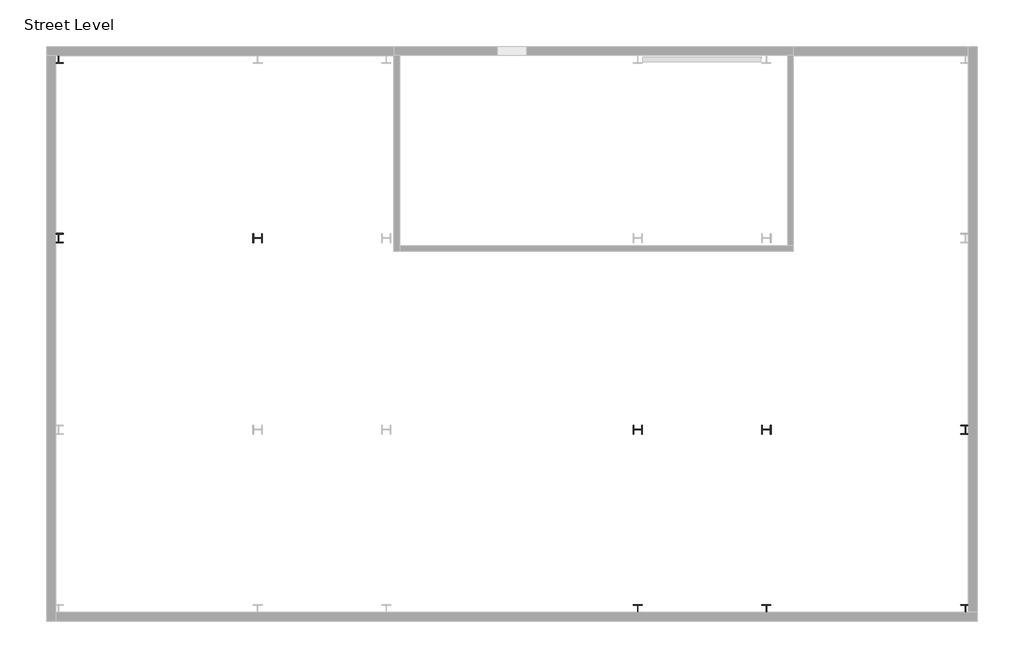
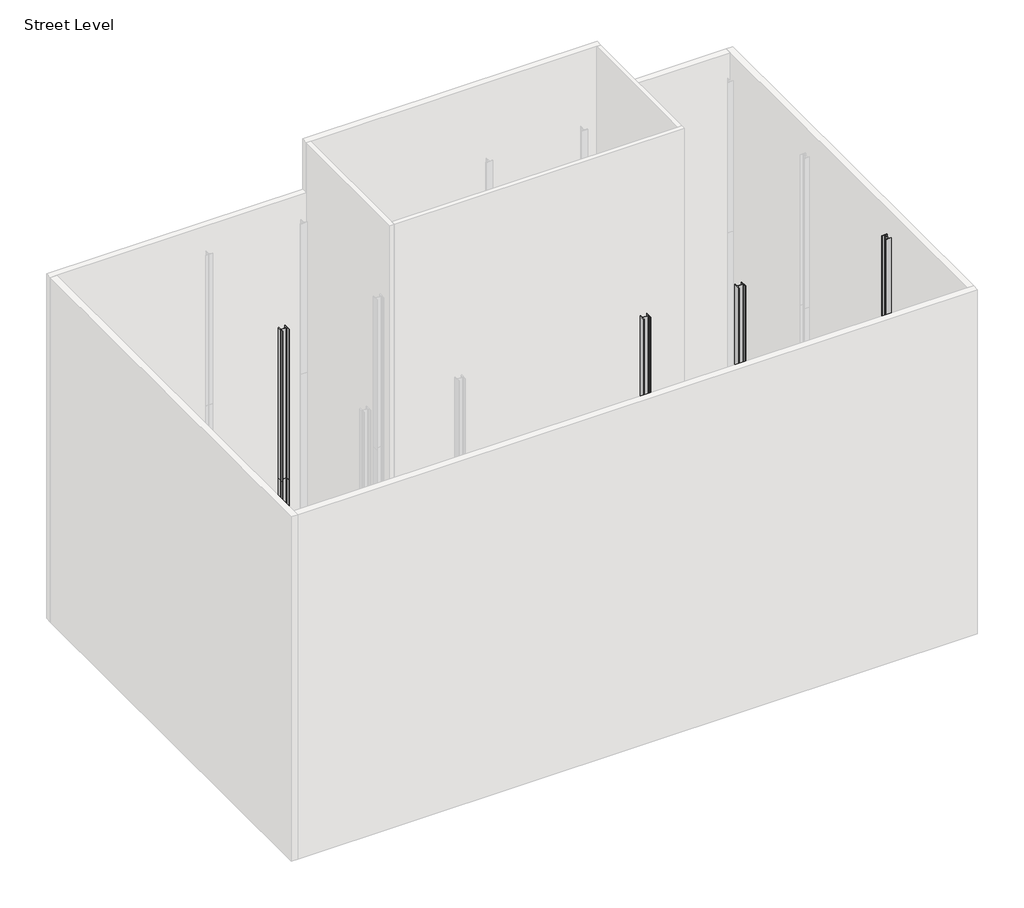
# One storey, part 2 of 3: 9 columns.
"""IFC4 building model written with IfcOpenShell, lengths in millimetres."""

from ifc_helpers import new_model, si_unit, point, frame, frame_2d, origin, place, context, project, spatial, polyline, circle_curve, trimmed, segment, composite_curve, outline, extrude, element, save

model = new_model("IFC4")

# Units and contexts
model_context = context("Model", 3, world=origin())
ifc_project = project(units=[si_unit("LENGTHUNIT", "METRE", prefix="MILLI")], contexts=[model_context])

# Site, building, storey
site = spatial("IfcSite", under=ifc_project)
building = spatial("IfcBuilding", under=site)
storey = spatial("IfcBuildingStorey", under=building, Name="Street Level", Elevation=-914.4)

# Columns
placement = place(None, origin())
element("IfcColumn", 1, ObjectType="W-Wide Flange-Column : W12X87", at=placement, inside=storey, context=model_context, shape_type="SweptSolid", body=[
    extrude(outline(composite_curve([segment(polyline([(3260.1377268, -3562.1684696), (3239.5637268, -3562.1684696), (3239.5637268, -3437.3274696)]), True, "CONTINUOUS"), segment(trimmed(circle_curve(frame_2d((3217.2752268, -3437.3274696)), 22.2885), [point((3239.5637268, -3437.3274696))], [point((3217.2752268, -3415.0389696))], True, "CARTESIAN"), True, "CONTINUOUS"), segment(polyline([(3217.2752268, -3415.0389696), (2985.5002268, -3415.0389696)]), True, "CONTINUOUS"), segment(trimmed(circle_curve(frame_2d((2985.5002268, -3437.3274696)), 22.2885), [point((2985.5002268, -3415.0389696))], [point((2963.2117268, -3437.3274696))], True, "CARTESIAN"), True, "CONTINUOUS"), segment(polyline([(2963.2117268, -3437.3274696), (2963.2117268, -3562.1684696), (2942.6377268, -3562.1684696), (2942.6377268, -3254.8284696), (2963.2117268, -3254.8284696), (2963.2117268, -3379.6694696)]), True, "CONTINUOUS"), segment(trimmed(circle_curve(frame_2d((2985.5002268, -3379.6694696)), 22.2885), [point((2963.2117268, -3379.6694696))], [point((2985.5002268, -3401.9579696))], True, "CARTESIAN"), True, "CONTINUOUS"), segment(polyline([(2985.5002268, -3401.9579696), (3217.2752268, -3401.9579696)]), True, "CONTINUOUS"), segment(trimmed(circle_curve(frame_2d((3217.2752268, -3379.6694696)), 22.2885), [point((3217.2752268, -3401.9579696))], [point((3239.5637268, -3379.6694696))], True, "CARTESIAN"), True, "CONTINUOUS"), segment(polyline([(3239.5637268, -3379.6694696), (3239.5637268, -3254.8284696), (3260.1377268, -3254.8284696), (3260.1377268, -3562.1684696)]), True, "CONTINUOUS")], self_intersect=False)), frame((0.0, 0.0, 7315.2), z_axis=(0.0, 0.0, 1.0), x_axis=(1.0, 0.0, 0.0)), (0.0, 0.0, 1.0), 7315.2),
    extrude(outline(composite_curve([segment(polyline([(3260.1377268, -3562.1684696), (3239.5637268, -3562.1684696), (3239.5637268, -3437.3274696)]), True, "CONTINUOUS"), segment(trimmed(circle_curve(frame_2d((3217.2752268, -3437.3274696)), 22.2885), [point((3239.5637268, -3437.3274696))], [point((3217.2752268, -3415.0389696))], True, "CARTESIAN"), True, "CONTINUOUS"), segment(polyline([(3217.2752268, -3415.0389696), (2985.5002268, -3415.0389696)]), True, "CONTINUOUS"), segment(trimmed(circle_curve(frame_2d((2985.5002268, -3437.3274696)), 22.2885), [point((2985.5002268, -3415.0389696))], [point((2963.2117268, -3437.3274696))], True, "CARTESIAN"), True, "CONTINUOUS"), segment(polyline([(2963.2117268, -3437.3274696), (2963.2117268, -3562.1684696), (2942.6377268, -3562.1684696), (2942.6377268, -3254.8284696), (2963.2117268, -3254.8284696), (2963.2117268, -3379.6694696)]), True, "CONTINUOUS"), segment(trimmed(circle_curve(frame_2d((2985.5002268, -3379.6694696)), 22.2885), [point((2963.2117268, -3379.6694696))], [point((2985.5002268, -3401.9579696))], True, "CARTESIAN"), True, "CONTINUOUS"), segment(polyline([(2985.5002268, -3401.9579696), (3217.2752268, -3401.9579696)]), True, "CONTINUOUS"), segment(trimmed(circle_curve(frame_2d((3217.2752268, -3379.6694696)), 22.2885), [point((3217.2752268, -3401.9579696))], [point((3239.5637268, -3379.6694696))], True, "CARTESIAN"), True, "CONTINUOUS"), segment(polyline([(3239.5637268, -3379.6694696), (3239.5637268, -3254.8284696), (3260.1377268, -3254.8284696), (3260.1377268, -3562.1684696)]), True, "CONTINUOUS")], self_intersect=False)), frame((0.0, 0.0, -914.4), z_axis=(0.0, 0.0, 1.0), x_axis=(1.0, 0.0, 0.0)), (0.0, 0.0, 1.0), 8229.6),
])
element("IfcColumn", 2, ObjectType="W-Wide Flange-Column : W12X87", at=placement, inside=storey, context=model_context, shape_type="SweptSolid", body=[
    extrude(outline(composite_curve([segment(polyline([(7628.9377268, -3562.1684696), (7608.3637268, -3562.1684696), (7608.3637268, -3437.3274696)]), True, "CONTINUOUS"), segment(trimmed(circle_curve(frame_2d((7586.0752268, -3437.3274696)), 22.2885), [point((7608.3637268, -3437.3274696))], [point((7586.0752268, -3415.0389696))], True, "CARTESIAN"), True, "CONTINUOUS"), segment(polyline([(7586.0752268, -3415.0389696), (7354.3002268, -3415.0389696)]), True, "CONTINUOUS"), segment(trimmed(circle_curve(frame_2d((7354.3002268, -3437.3274696)), 22.2885), [point((7354.3002268, -3415.0389696))], [point((7332.0117268, -3437.3274696))], True, "CARTESIAN"), True, "CONTINUOUS"), segment(polyline([(7332.0117268, -3437.3274696), (7332.0117268, -3562.1684696), (7311.4377268, -3562.1684696), (7311.4377268, -3254.8284696), (7332.0117268, -3254.8284696), (7332.0117268, -3379.6694696)]), True, "CONTINUOUS"), segment(trimmed(circle_curve(frame_2d((7354.3002268, -3379.6694696)), 22.2885), [point((7332.0117268, -3379.6694696))], [point((7354.3002268, -3401.9579696))], True, "CARTESIAN"), True, "CONTINUOUS"), segment(polyline([(7354.3002268, -3401.9579696), (7586.0752268, -3401.9579696)]), True, "CONTINUOUS"), segment(trimmed(circle_curve(frame_2d((7586.0752268, -3379.6694696)), 22.2885), [point((7586.0752268, -3401.9579696))], [point((7608.3637268, -3379.6694696))], True, "CARTESIAN"), True, "CONTINUOUS"), segment(polyline([(7608.3637268, -3379.6694696), (7608.3637268, -3254.8284696), (7628.9377268, -3254.8284696), (7628.9377268, -3562.1684696)]), True, "CONTINUOUS")], self_intersect=False)), frame((0.0, 0.0, 7315.2), z_axis=(0.0, 0.0, 1.0), x_axis=(1.0, 0.0, 0.0)), (0.0, 0.0, 1.0), 7315.2),
    extrude(outline(composite_curve([segment(polyline([(7628.9377268, -3562.1684696), (7608.3637268, -3562.1684696), (7608.3637268, -3437.3274696)]), True, "CONTINUOUS"), segment(trimmed(circle_curve(frame_2d((7586.0752268, -3437.3274696)), 22.2885), [point((7608.3637268, -3437.3274696))], [point((7586.0752268, -3415.0389696))], True, "CARTESIAN"), True, "CONTINUOUS"), segment(polyline([(7586.0752268, -3415.0389696), (7354.3002268, -3415.0389696)]), True, "CONTINUOUS"), segment(trimmed(circle_curve(frame_2d((7354.3002268, -3437.3274696)), 22.2885), [point((7354.3002268, -3415.0389696))], [point((7332.0117268, -3437.3274696))], True, "CARTESIAN"), True, "CONTINUOUS"), segment(polyline([(7332.0117268, -3437.3274696), (7332.0117268, -3562.1684696), (7311.4377268, -3562.1684696), (7311.4377268, -3254.8284696), (7332.0117268, -3254.8284696), (7332.0117268, -3379.6694696)]), True, "CONTINUOUS"), segment(trimmed(circle_curve(frame_2d((7354.3002268, -3379.6694696)), 22.2885), [point((7332.0117268, -3379.6694696))], [point((7354.3002268, -3401.9579696))], True, "CARTESIAN"), True, "CONTINUOUS"), segment(polyline([(7354.3002268, -3401.9579696), (7586.0752268, -3401.9579696)]), True, "CONTINUOUS"), segment(trimmed(circle_curve(frame_2d((7586.0752268, -3379.6694696)), 22.2885), [point((7586.0752268, -3401.9579696))], [point((7608.3637268, -3379.6694696))], True, "CARTESIAN"), True, "CONTINUOUS"), segment(polyline([(7608.3637268, -3379.6694696), (7608.3637268, -3254.8284696), (7628.9377268, -3254.8284696), (7628.9377268, -3562.1684696)]), True, "CONTINUOUS")], self_intersect=False)), frame((0.0, 0.0, -914.4), z_axis=(0.0, 0.0, 1.0), x_axis=(1.0, 0.0, 0.0)), (0.0, 0.0, 1.0), 8229.6),
])
element("IfcColumn", 3, ObjectType="W-Wide Flange-Column : W12X87", at=placement, inside=storey, context=model_context, shape_type="SweptSolid", body=[
    extrude(outline(composite_curve([segment(polyline([(-9643.0622732, 2940.2315304), (-9663.6362732, 2940.2315304), (-9663.6362732, 3065.0725304)]), True, "CONTINUOUS"), segment(trimmed(circle_curve(frame_2d((-9685.9247732, 3065.0725304)), 22.2885), [point((-9663.6362732, 3065.0725304))], [point((-9685.9247732, 3087.3610304))], True, "CARTESIAN"), True, "CONTINUOUS"), segment(polyline([(-9685.9247732, 3087.3610304), (-9917.6997732, 3087.3610304)]), True, "CONTINUOUS"), segment(trimmed(circle_curve(frame_2d((-9917.6997732, 3065.0725304)), 22.2885), [point((-9917.6997732, 3087.3610304))], [point((-9939.9882732, 3065.0725304))], True, "CARTESIAN"), True, "CONTINUOUS"), segment(polyline([(-9939.9882732, 3065.0725304), (-9939.9882732, 2940.2315304), (-9960.5622732, 2940.2315304), (-9960.5622732, 3247.5715304), (-9939.9882732, 3247.5715304), (-9939.9882732, 3122.7305304)]), True, "CONTINUOUS"), segment(trimmed(circle_curve(frame_2d((-9917.6997732, 3122.7305304)), 22.2885), [point((-9939.9882732, 3122.7305304))], [point((-9917.6997732, 3100.4420304))], True, "CARTESIAN"), True, "CONTINUOUS"), segment(polyline([(-9917.6997732, 3100.4420304), (-9685.9247732, 3100.4420304)]), True, "CONTINUOUS"), segment(trimmed(circle_curve(frame_2d((-9685.9247732, 3122.7305304)), 22.2885), [point((-9685.9247732, 3100.4420304))], [point((-9663.6362732, 3122.7305304))], True, "CARTESIAN"), True, "CONTINUOUS"), segment(polyline([(-9663.6362732, 3122.7305304), (-9663.6362732, 3247.5715304), (-9643.0622732, 3247.5715304), (-9643.0622732, 2940.2315304)]), True, "CONTINUOUS")], self_intersect=False)), frame((0.0, 0.0, 7315.2), z_axis=(0.0, 0.0, 1.0), x_axis=(1.0, 0.0, 0.0)), (0.0, 0.0, 1.0), 7315.2),
    extrude(outline(composite_curve([segment(polyline([(-9643.0622732, 2940.2315304), (-9663.6362732, 2940.2315304), (-9663.6362732, 3065.0725304)]), True, "CONTINUOUS"), segment(trimmed(circle_curve(frame_2d((-9685.9247732, 3065.0725304)), 22.2885), [point((-9663.6362732, 3065.0725304))], [point((-9685.9247732, 3087.3610304))], True, "CARTESIAN"), True, "CONTINUOUS"), segment(polyline([(-9685.9247732, 3087.3610304), (-9917.6997732, 3087.3610304)]), True, "CONTINUOUS"), segment(trimmed(circle_curve(frame_2d((-9917.6997732, 3065.0725304)), 22.2885), [point((-9917.6997732, 3087.3610304))], [point((-9939.9882732, 3065.0725304))], True, "CARTESIAN"), True, "CONTINUOUS"), segment(polyline([(-9939.9882732, 3065.0725304), (-9939.9882732, 2940.2315304), (-9960.5622732, 2940.2315304), (-9960.5622732, 3247.5715304), (-9939.9882732, 3247.5715304), (-9939.9882732, 3122.7305304)]), True, "CONTINUOUS"), segment(trimmed(circle_curve(frame_2d((-9917.6997732, 3122.7305304)), 22.2885), [point((-9939.9882732, 3122.7305304))], [point((-9917.6997732, 3100.4420304))], True, "CARTESIAN"), True, "CONTINUOUS"), segment(polyline([(-9917.6997732, 3100.4420304), (-9685.9247732, 3100.4420304)]), True, "CONTINUOUS"), segment(trimmed(circle_curve(frame_2d((-9685.9247732, 3122.7305304)), 22.2885), [point((-9685.9247732, 3100.4420304))], [point((-9663.6362732, 3122.7305304))], True, "CARTESIAN"), True, "CONTINUOUS"), segment(polyline([(-9663.6362732, 3122.7305304), (-9663.6362732, 3247.5715304), (-9643.0622732, 3247.5715304), (-9643.0622732, 2940.2315304)]), True, "CONTINUOUS")], self_intersect=False)), frame((0.0, 0.0, -914.4), z_axis=(0.0, 0.0, 1.0), x_axis=(1.0, 0.0, 0.0)), (0.0, 0.0, 1.0), 8229.6),
])
element("IfcColumn", 4, ObjectType="W-Wide Flange-Column : W12X87", at=placement, inside=storey, context=model_context, shape_type="SweptSolid", body=[
    extrude(outline(composite_curve([segment(polyline([(-16404.5422732, 9348.6515304), (-16404.5422732, 9328.0775304), (-16529.3832732, 9328.0775304)]), True, "CONTINUOUS"), segment(trimmed(circle_curve(frame_2d((-16529.3832732, 9305.7890304)), 22.2885), [point((-16529.3832732, 9328.0775304))], [point((-16551.6717732, 9305.7890304))], True, "CARTESIAN"), True, "CONTINUOUS"), segment(polyline([(-16551.6717732, 9305.7890304), (-16551.6717732, 9074.0140304)]), True, "CONTINUOUS"), segment(trimmed(circle_curve(frame_2d((-16529.3832732, 9074.0140304)), 22.2885), [point((-16551.6717732, 9074.0140304))], [point((-16529.3832732, 9051.7255304))], True, "CARTESIAN"), True, "CONTINUOUS"), segment(polyline([(-16529.3832732, 9051.7255304), (-16404.5422732, 9051.7255304), (-16404.5422732, 9031.1515304), (-16711.8822732, 9031.1515304), (-16711.8822732, 9051.7255304), (-16587.0412732, 9051.7255304)]), True, "CONTINUOUS"), segment(trimmed(circle_curve(frame_2d((-16587.0412732, 9074.0140304)), 22.2885), [point((-16587.0412732, 9051.7255304))], [point((-16564.7527732, 9074.0140304))], True, "CARTESIAN"), True, "CONTINUOUS"), segment(polyline([(-16564.7527732, 9074.0140304), (-16564.7527732, 9305.7890304)]), True, "CONTINUOUS"), segment(trimmed(circle_curve(frame_2d((-16587.0412732, 9305.7890304)), 22.2885), [point((-16564.7527732, 9305.7890304))], [point((-16587.0412732, 9328.0775304))], True, "CARTESIAN"), True, "CONTINUOUS"), segment(polyline([(-16587.0412732, 9328.0775304), (-16711.8822732, 9328.0775304), (-16711.8822732, 9348.6515304), (-16404.5422732, 9348.6515304)]), True, "CONTINUOUS")], self_intersect=False)), frame((0.0, 0.0, 7315.2), z_axis=(0.0, 0.0, 1.0), x_axis=(1.0, 0.0, 0.0)), (0.0, 0.0, 1.0), 7315.2),
    extrude(outline(composite_curve([segment(polyline([(-16404.5422732, 9348.6515304), (-16404.5422732, 9328.0775304), (-16529.3832732, 9328.0775304)]), True, "CONTINUOUS"), segment(trimmed(circle_curve(frame_2d((-16529.3832732, 9305.7890304)), 22.2885), [point((-16529.3832732, 9328.0775304))], [point((-16551.6717732, 9305.7890304))], True, "CARTESIAN"), True, "CONTINUOUS"), segment(polyline([(-16551.6717732, 9305.7890304), (-16551.6717732, 9074.0140304)]), True, "CONTINUOUS"), segment(trimmed(circle_curve(frame_2d((-16529.3832732, 9074.0140304)), 22.2885), [point((-16551.6717732, 9074.0140304))], [point((-16529.3832732, 9051.7255304))], True, "CARTESIAN"), True, "CONTINUOUS"), segment(polyline([(-16529.3832732, 9051.7255304), (-16404.5422732, 9051.7255304), (-16404.5422732, 9031.1515304), (-16711.8822732, 9031.1515304), (-16711.8822732, 9051.7255304), (-16587.0412732, 9051.7255304)]), True, "CONTINUOUS"), segment(trimmed(circle_curve(frame_2d((-16587.0412732, 9074.0140304)), 22.2885), [point((-16587.0412732, 9051.7255304))], [point((-16564.7527732, 9074.0140304))], True, "CARTESIAN"), True, "CONTINUOUS"), segment(polyline([(-16564.7527732, 9074.0140304), (-16564.7527732, 9305.7890304)]), True, "CONTINUOUS"), segment(trimmed(circle_curve(frame_2d((-16587.0412732, 9305.7890304)), 22.2885), [point((-16564.7527732, 9305.7890304))], [point((-16587.0412732, 9328.0775304))], True, "CARTESIAN"), True, "CONTINUOUS"), segment(polyline([(-16587.0412732, 9328.0775304), (-16711.8822732, 9328.0775304), (-16711.8822732, 9348.6515304), (-16404.5422732, 9348.6515304)]), True, "CONTINUOUS")], self_intersect=False)), frame((0.0, 0.0, -914.4), z_axis=(0.0, 0.0, 1.0), x_axis=(1.0, 0.0, 0.0)), (0.0, 0.0, 1.0), 8229.6),
])
element("IfcColumn", 5, ObjectType="W-Wide Flange-Column : W12X87", at=placement, inside=storey, context=model_context, shape_type="SweptSolid", body=[
    extrude(outline(composite_curve([segment(polyline([(-16404.5422732, 3252.6515304), (-16404.5422732, 3232.0775304), (-16529.3832732, 3232.0775304)]), True, "CONTINUOUS"), segment(trimmed(circle_curve(frame_2d((-16529.3832732, 3209.7890304)), 22.2885), [point((-16529.3832732, 3232.0775304))], [point((-16551.6717732, 3209.7890304))], True, "CARTESIAN"), True, "CONTINUOUS"), segment(polyline([(-16551.6717732, 3209.7890304), (-16551.6717732, 2978.0140304)]), True, "CONTINUOUS"), segment(trimmed(circle_curve(frame_2d((-16529.3832732, 2978.0140304)), 22.2885), [point((-16551.6717732, 2978.0140304))], [point((-16529.3832732, 2955.7255304))], True, "CARTESIAN"), True, "CONTINUOUS"), segment(polyline([(-16529.3832732, 2955.7255304), (-16404.5422732, 2955.7255304), (-16404.5422732, 2935.1515304), (-16711.8822732, 2935.1515304), (-16711.8822732, 2955.7255304), (-16587.0412732, 2955.7255304)]), True, "CONTINUOUS"), segment(trimmed(circle_curve(frame_2d((-16587.0412732, 2978.0140304)), 22.2885), [point((-16587.0412732, 2955.7255304))], [point((-16564.7527732, 2978.0140304))], True, "CARTESIAN"), True, "CONTINUOUS"), segment(polyline([(-16564.7527732, 2978.0140304), (-16564.7527732, 3209.7890304)]), True, "CONTINUOUS"), segment(trimmed(circle_curve(frame_2d((-16587.0412732, 3209.7890304)), 22.2885), [point((-16564.7527732, 3209.7890304))], [point((-16587.0412732, 3232.0775304))], True, "CARTESIAN"), True, "CONTINUOUS"), segment(polyline([(-16587.0412732, 3232.0775304), (-16711.8822732, 3232.0775304), (-16711.8822732, 3252.6515304), (-16404.5422732, 3252.6515304)]), True, "CONTINUOUS")], self_intersect=False)), frame((0.0, 0.0, 7315.2), z_axis=(0.0, 0.0, 1.0), x_axis=(1.0, 0.0, 0.0)), (0.0, 0.0, 1.0), 7315.2),
    extrude(outline(composite_curve([segment(polyline([(-16404.5422732, 3252.6515304), (-16404.5422732, 3232.0775304), (-16529.3832732, 3232.0775304)]), True, "CONTINUOUS"), segment(trimmed(circle_curve(frame_2d((-16529.3832732, 3209.7890304)), 22.2885), [point((-16529.3832732, 3232.0775304))], [point((-16551.6717732, 3209.7890304))], True, "CARTESIAN"), True, "CONTINUOUS"), segment(polyline([(-16551.6717732, 3209.7890304), (-16551.6717732, 2978.0140304)]), True, "CONTINUOUS"), segment(trimmed(circle_curve(frame_2d((-16529.3832732, 2978.0140304)), 22.2885), [point((-16551.6717732, 2978.0140304))], [point((-16529.3832732, 2955.7255304))], True, "CARTESIAN"), True, "CONTINUOUS"), segment(polyline([(-16529.3832732, 2955.7255304), (-16404.5422732, 2955.7255304), (-16404.5422732, 2935.1515304), (-16711.8822732, 2935.1515304), (-16711.8822732, 2955.7255304), (-16587.0412732, 2955.7255304)]), True, "CONTINUOUS"), segment(trimmed(circle_curve(frame_2d((-16587.0412732, 2978.0140304)), 22.2885), [point((-16587.0412732, 2955.7255304))], [point((-16564.7527732, 2978.0140304))], True, "CARTESIAN"), True, "CONTINUOUS"), segment(polyline([(-16564.7527732, 2978.0140304), (-16564.7527732, 3209.7890304)]), True, "CONTINUOUS"), segment(trimmed(circle_curve(frame_2d((-16587.0412732, 3209.7890304)), 22.2885), [point((-16564.7527732, 3209.7890304))], [point((-16587.0412732, 3232.0775304))], True, "CARTESIAN"), True, "CONTINUOUS"), segment(polyline([(-16587.0412732, 3232.0775304), (-16711.8822732, 3232.0775304), (-16711.8822732, 3252.6515304), (-16404.5422732, 3252.6515304)]), True, "CONTINUOUS")], self_intersect=False)), frame((0.0, 0.0, -914.4), z_axis=(0.0, 0.0, 1.0), x_axis=(1.0, 0.0, 0.0)), (0.0, 0.0, 1.0), 8229.6),
])
element("IfcColumn", 6, ObjectType="W-Wide Flange-Column : W12X87", at=placement, inside=storey, context=model_context, shape_type="SweptSolid", body=[
    extrude(outline(composite_curve([segment(polyline([(14380.2577268, -3249.7484696), (14380.2577268, -3270.3224696), (14255.4167268, -3270.3224696)]), True, "CONTINUOUS"), segment(trimmed(circle_curve(frame_2d((14255.4167268, -3292.6109696)), 22.2885), [point((14255.4167268, -3270.3224696))], [point((14233.1282268, -3292.6109696))], True, "CARTESIAN"), True, "CONTINUOUS"), segment(polyline([(14233.1282268, -3292.6109696), (14233.1282268, -3524.3859696)]), True, "CONTINUOUS"), segment(trimmed(circle_curve(frame_2d((14255.4167268, -3524.3859696)), 22.2885), [point((14233.1282268, -3524.3859696))], [point((14255.4167268, -3546.6744696))], True, "CARTESIAN"), True, "CONTINUOUS"), segment(polyline([(14255.4167268, -3546.6744696), (14380.2577268, -3546.6744696), (14380.2577268, -3567.2484696), (14072.9177268, -3567.2484696), (14072.9177268, -3546.6744696), (14197.7587268, -3546.6744696)]), True, "CONTINUOUS"), segment(trimmed(circle_curve(frame_2d((14197.7587268, -3524.3859696)), 22.2885), [point((14197.7587268, -3546.6744696))], [point((14220.0472268, -3524.3859696))], True, "CARTESIAN"), True, "CONTINUOUS"), segment(polyline([(14220.0472268, -3524.3859696), (14220.0472268, -3292.6109696)]), True, "CONTINUOUS"), segment(trimmed(circle_curve(frame_2d((14197.7587268, -3292.6109696)), 22.2885), [point((14220.0472268, -3292.6109696))], [point((14197.7587268, -3270.3224696))], True, "CARTESIAN"), True, "CONTINUOUS"), segment(polyline([(14197.7587268, -3270.3224696), (14072.9177268, -3270.3224696), (14072.9177268, -3249.7484696), (14380.2577268, -3249.7484696)]), True, "CONTINUOUS")], self_intersect=False)), frame((0.0, 0.0, 7315.2), z_axis=(0.0, 0.0, 1.0), x_axis=(1.0, 0.0, 0.0)), (0.0, 0.0, 1.0), 7315.2),
    extrude(outline(composite_curve([segment(polyline([(14380.2577268, -3249.7484696), (14380.2577268, -3270.3224696), (14255.4167268, -3270.3224696)]), True, "CONTINUOUS"), segment(trimmed(circle_curve(frame_2d((14255.4167268, -3292.6109696)), 22.2885), [point((14255.4167268, -3270.3224696))], [point((14233.1282268, -3292.6109696))], True, "CARTESIAN"), True, "CONTINUOUS"), segment(polyline([(14233.1282268, -3292.6109696), (14233.1282268, -3524.3859696)]), True, "CONTINUOUS"), segment(trimmed(circle_curve(frame_2d((14255.4167268, -3524.3859696)), 22.2885), [point((14233.1282268, -3524.3859696))], [point((14255.4167268, -3546.6744696))], True, "CARTESIAN"), True, "CONTINUOUS"), segment(polyline([(14255.4167268, -3546.6744696), (14380.2577268, -3546.6744696), (14380.2577268, -3567.2484696), (14072.9177268, -3567.2484696), (14072.9177268, -3546.6744696), (14197.7587268, -3546.6744696)]), True, "CONTINUOUS"), segment(trimmed(circle_curve(frame_2d((14197.7587268, -3524.3859696)), 22.2885), [point((14197.7587268, -3546.6744696))], [point((14220.0472268, -3524.3859696))], True, "CARTESIAN"), True, "CONTINUOUS"), segment(polyline([(14220.0472268, -3524.3859696), (14220.0472268, -3292.6109696)]), True, "CONTINUOUS"), segment(trimmed(circle_curve(frame_2d((14197.7587268, -3292.6109696)), 22.2885), [point((14220.0472268, -3292.6109696))], [point((14197.7587268, -3270.3224696))], True, "CARTESIAN"), True, "CONTINUOUS"), segment(polyline([(14197.7587268, -3270.3224696), (14072.9177268, -3270.3224696), (14072.9177268, -3249.7484696), (14380.2577268, -3249.7484696)]), True, "CONTINUOUS")], self_intersect=False)), frame((0.0, 0.0, -914.4), z_axis=(0.0, 0.0, 1.0), x_axis=(1.0, 0.0, 0.0)), (0.0, 0.0, 1.0), 8229.6),
])
element("IfcColumn", 7, ObjectType="W-Wide Flange-Column : W12X87", at=placement, inside=storey, context=model_context, shape_type="SweptSolid", body=[
    extrude(outline(composite_curve([segment(polyline([(14380.2577268, -9345.7484696), (14380.2577268, -9366.3224696), (14255.4167268, -9366.3224696)]), True, "CONTINUOUS"), segment(trimmed(circle_curve(frame_2d((14255.4167268, -9388.6109696)), 22.2885), [point((14255.4167268, -9366.3224696))], [point((14233.1282268, -9388.6109696))], True, "CARTESIAN"), True, "CONTINUOUS"), segment(polyline([(14233.1282268, -9388.6109696), (14233.1282268, -9620.3859696)]), True, "CONTINUOUS"), segment(trimmed(circle_curve(frame_2d((14255.4167268, -9620.3859696)), 22.2885), [point((14233.1282268, -9620.3859696))], [point((14255.4167268, -9642.6744696))], True, "CARTESIAN"), True, "CONTINUOUS"), segment(polyline([(14255.4167268, -9642.6744696), (14380.2577268, -9642.6744696), (14380.2577268, -9663.2484696), (14072.9177268, -9663.2484696), (14072.9177268, -9642.6744696), (14197.7587268, -9642.6744696)]), True, "CONTINUOUS"), segment(trimmed(circle_curve(frame_2d((14197.7587268, -9620.3859696)), 22.2885), [point((14197.7587268, -9642.6744696))], [point((14220.0472268, -9620.3859696))], True, "CARTESIAN"), True, "CONTINUOUS"), segment(polyline([(14220.0472268, -9620.3859696), (14220.0472268, -9388.6109696)]), True, "CONTINUOUS"), segment(trimmed(circle_curve(frame_2d((14197.7587268, -9388.6109696)), 22.2885), [point((14220.0472268, -9388.6109696))], [point((14197.7587268, -9366.3224696))], True, "CARTESIAN"), True, "CONTINUOUS"), segment(polyline([(14197.7587268, -9366.3224696), (14072.9177268, -9366.3224696), (14072.9177268, -9345.7484696), (14380.2577268, -9345.7484696)]), True, "CONTINUOUS")], self_intersect=False)), frame((0.0, 0.0, 7315.2), z_axis=(0.0, 0.0, 1.0), x_axis=(1.0, 0.0, 0.0)), (0.0, 0.0, 1.0), 7315.2),
    extrude(outline(composite_curve([segment(polyline([(14380.2577268, -9345.7484696), (14380.2577268, -9366.3224696), (14255.4167268, -9366.3224696)]), True, "CONTINUOUS"), segment(trimmed(circle_curve(frame_2d((14255.4167268, -9388.6109696)), 22.2885), [point((14255.4167268, -9366.3224696))], [point((14233.1282268, -9388.6109696))], True, "CARTESIAN"), True, "CONTINUOUS"), segment(polyline([(14233.1282268, -9388.6109696), (14233.1282268, -9620.3859696)]), True, "CONTINUOUS"), segment(trimmed(circle_curve(frame_2d((14255.4167268, -9620.3859696)), 22.2885), [point((14233.1282268, -9620.3859696))], [point((14255.4167268, -9642.6744696))], True, "CARTESIAN"), True, "CONTINUOUS"), segment(polyline([(14255.4167268, -9642.6744696), (14380.2577268, -9642.6744696), (14380.2577268, -9663.2484696), (14072.9177268, -9663.2484696), (14072.9177268, -9642.6744696), (14197.7587268, -9642.6744696)]), True, "CONTINUOUS"), segment(trimmed(circle_curve(frame_2d((14197.7587268, -9620.3859696)), 22.2885), [point((14197.7587268, -9642.6744696))], [point((14220.0472268, -9620.3859696))], True, "CARTESIAN"), True, "CONTINUOUS"), segment(polyline([(14220.0472268, -9620.3859696), (14220.0472268, -9388.6109696)]), True, "CONTINUOUS"), segment(trimmed(circle_curve(frame_2d((14197.7587268, -9388.6109696)), 22.2885), [point((14220.0472268, -9388.6109696))], [point((14197.7587268, -9366.3224696))], True, "CARTESIAN"), True, "CONTINUOUS"), segment(polyline([(14197.7587268, -9366.3224696), (14072.9177268, -9366.3224696), (14072.9177268, -9345.7484696), (14380.2577268, -9345.7484696)]), True, "CONTINUOUS")], self_intersect=False)), frame((0.0, 0.0, -914.4), z_axis=(0.0, 0.0, 1.0), x_axis=(1.0, 0.0, 0.0)), (0.0, 0.0, 1.0), 8229.6),
])
element("IfcColumn", 8, ObjectType="W-Wide Flange-Column : W12X87", at=placement, inside=storey, context=model_context, shape_type="SweptSolid", body=[
    extrude(outline(composite_curve([segment(polyline([(7623.8577268, -9345.7484696), (7623.8577268, -9366.3224696), (7499.0167268, -9366.3224696)]), True, "CONTINUOUS"), segment(trimmed(circle_curve(frame_2d((7499.0167268, -9388.6109696)), 22.2885), [point((7499.0167268, -9366.3224696))], [point((7476.7282268, -9388.6109696))], True, "CARTESIAN"), True, "CONTINUOUS"), segment(polyline([(7476.7282268, -9388.6109696), (7476.7282268, -9620.3859696)]), True, "CONTINUOUS"), segment(trimmed(circle_curve(frame_2d((7499.0167268, -9620.3859696)), 22.2885), [point((7476.7282268, -9620.3859696))], [point((7499.0167268, -9642.6744696))], True, "CARTESIAN"), True, "CONTINUOUS"), segment(polyline([(7499.0167268, -9642.6744696), (7623.8577268, -9642.6744696), (7623.8577268, -9663.2484696), (7316.5177268, -9663.2484696), (7316.5177268, -9642.6744696), (7441.3587268, -9642.6744696)]), True, "CONTINUOUS"), segment(trimmed(circle_curve(frame_2d((7441.3587268, -9620.3859696)), 22.2885), [point((7441.3587268, -9642.6744696))], [point((7463.6472268, -9620.3859696))], True, "CARTESIAN"), True, "CONTINUOUS"), segment(polyline([(7463.6472268, -9620.3859696), (7463.6472268, -9388.6109696)]), True, "CONTINUOUS"), segment(trimmed(circle_curve(frame_2d((7441.3587268, -9388.6109696)), 22.2885), [point((7463.6472268, -9388.6109696))], [point((7441.3587268, -9366.3224696))], True, "CARTESIAN"), True, "CONTINUOUS"), segment(polyline([(7441.3587268, -9366.3224696), (7316.5177268, -9366.3224696), (7316.5177268, -9345.7484696), (7623.8577268, -9345.7484696)]), True, "CONTINUOUS")], self_intersect=False)), frame((0.0, 0.0, 7315.2), z_axis=(0.0, 0.0, 1.0), x_axis=(1.0, 0.0, 0.0)), (0.0, 0.0, 1.0), 7315.2),
    extrude(outline(composite_curve([segment(polyline([(7623.8577268, -9345.7484696), (7623.8577268, -9366.3224696), (7499.0167268, -9366.3224696)]), True, "CONTINUOUS"), segment(trimmed(circle_curve(frame_2d((7499.0167268, -9388.6109696)), 22.2885), [point((7499.0167268, -9366.3224696))], [point((7476.7282268, -9388.6109696))], True, "CARTESIAN"), True, "CONTINUOUS"), segment(polyline([(7476.7282268, -9388.6109696), (7476.7282268, -9620.3859696)]), True, "CONTINUOUS"), segment(trimmed(circle_curve(frame_2d((7499.0167268, -9620.3859696)), 22.2885), [point((7476.7282268, -9620.3859696))], [point((7499.0167268, -9642.6744696))], True, "CARTESIAN"), True, "CONTINUOUS"), segment(polyline([(7499.0167268, -9642.6744696), (7623.8577268, -9642.6744696), (7623.8577268, -9663.2484696), (7316.5177268, -9663.2484696), (7316.5177268, -9642.6744696), (7441.3587268, -9642.6744696)]), True, "CONTINUOUS"), segment(trimmed(circle_curve(frame_2d((7441.3587268, -9620.3859696)), 22.2885), [point((7441.3587268, -9642.6744696))], [point((7463.6472268, -9620.3859696))], True, "CARTESIAN"), True, "CONTINUOUS"), segment(polyline([(7463.6472268, -9620.3859696), (7463.6472268, -9388.6109696)]), True, "CONTINUOUS"), segment(trimmed(circle_curve(frame_2d((7441.3587268, -9388.6109696)), 22.2885), [point((7463.6472268, -9388.6109696))], [point((7441.3587268, -9366.3224696))], True, "CARTESIAN"), True, "CONTINUOUS"), segment(polyline([(7441.3587268, -9366.3224696), (7316.5177268, -9366.3224696), (7316.5177268, -9345.7484696), (7623.8577268, -9345.7484696)]), True, "CONTINUOUS")], self_intersect=False)), frame((0.0, 0.0, -914.4), z_axis=(0.0, 0.0, 1.0), x_axis=(1.0, 0.0, 0.0)), (0.0, 0.0, 1.0), 8229.6),
])
element("IfcColumn", 9, ObjectType="W-Wide Flange-Column : W12X87", at=placement, inside=storey, context=model_context, shape_type="SweptSolid", body=[
    extrude(outline(composite_curve([segment(polyline([(3255.0577268, -9345.7484696), (3255.0577268, -9366.3224696), (3130.2167268, -9366.3224696)]), True, "CONTINUOUS"), segment(trimmed(circle_curve(frame_2d((3130.2167268, -9388.6109696)), 22.2885), [point((3130.2167268, -9366.3224696))], [point((3107.9282268, -9388.6109696))], True, "CARTESIAN"), True, "CONTINUOUS"), segment(polyline([(3107.9282268, -9388.6109696), (3107.9282268, -9620.3859696)]), True, "CONTINUOUS"), segment(trimmed(circle_curve(frame_2d((3130.2167268, -9620.3859696)), 22.2885), [point((3107.9282268, -9620.3859696))], [point((3130.2167268, -9642.6744696))], True, "CARTESIAN"), True, "CONTINUOUS"), segment(polyline([(3130.2167268, -9642.6744696), (3255.0577268, -9642.6744696), (3255.0577268, -9663.2484696), (2947.7177268, -9663.2484696), (2947.7177268, -9642.6744696), (3072.5587268, -9642.6744696)]), True, "CONTINUOUS"), segment(trimmed(circle_curve(frame_2d((3072.5587268, -9620.3859696)), 22.2885), [point((3072.5587268, -9642.6744696))], [point((3094.8472268, -9620.3859696))], True, "CARTESIAN"), True, "CONTINUOUS"), segment(polyline([(3094.8472268, -9620.3859696), (3094.8472268, -9388.6109696)]), True, "CONTINUOUS"), segment(trimmed(circle_curve(frame_2d((3072.5587268, -9388.6109696)), 22.2885), [point((3094.8472268, -9388.6109696))], [point((3072.5587268, -9366.3224696))], True, "CARTESIAN"), True, "CONTINUOUS"), segment(polyline([(3072.5587268, -9366.3224696), (2947.7177268, -9366.3224696), (2947.7177268, -9345.7484696), (3255.0577268, -9345.7484696)]), True, "CONTINUOUS")], self_intersect=False)), frame((0.0, 0.0, 7315.2), z_axis=(0.0, 0.0, 1.0), x_axis=(1.0, 0.0, 0.0)), (0.0, 0.0, 1.0), 7315.2),
    extrude(outline(composite_curve([segment(polyline([(3255.0577268, -9345.7484696), (3255.0577268, -9366.3224696), (3130.2167268, -9366.3224696)]), True, "CONTINUOUS"), segment(trimmed(circle_curve(frame_2d((3130.2167268, -9388.6109696)), 22.2885), [point((3130.2167268, -9366.3224696))], [point((3107.9282268, -9388.6109696))], True, "CARTESIAN"), True, "CONTINUOUS"), segment(polyline([(3107.9282268, -9388.6109696), (3107.9282268, -9620.3859696)]), True, "CONTINUOUS"), segment(trimmed(circle_curve(frame_2d((3130.2167268, -9620.3859696)), 22.2885), [point((3107.9282268, -9620.3859696))], [point((3130.2167268, -9642.6744696))], True, "CARTESIAN"), True, "CONTINUOUS"), segment(polyline([(3130.2167268, -9642.6744696), (3255.0577268, -9642.6744696), (3255.0577268, -9663.2484696), (2947.7177268, -9663.2484696), (2947.7177268, -9642.6744696), (3072.5587268, -9642.6744696)]), True, "CONTINUOUS"), segment(trimmed(circle_curve(frame_2d((3072.5587268, -9620.3859696)), 22.2885), [point((3072.5587268, -9642.6744696))], [point((3094.8472268, -9620.3859696))], True, "CARTESIAN"), True, "CONTINUOUS"), segment(polyline([(3094.8472268, -9620.3859696), (3094.8472268, -9388.6109696)]), True, "CONTINUOUS"), segment(trimmed(circle_curve(frame_2d((3072.5587268, -9388.6109696)), 22.2885), [point((3094.8472268, -9388.6109696))], [point((3072.5587268, -9366.3224696))], True, "CARTESIAN"), True, "CONTINUOUS"), segment(polyline([(3072.5587268, -9366.3224696), (2947.7177268, -9366.3224696), (2947.7177268, -9345.7484696), (3255.0577268, -9345.7484696)]), True, "CONTINUOUS")], self_intersect=False)), frame((0.0, 0.0, -914.4), z_axis=(0.0, 0.0, 1.0), x_axis=(1.0, 0.0, 0.0)), (0.0, 0.0, 1.0), 8229.6),
])

save(model, "model.ifc")

# Revit data of these elements
# Type "W-Wide Flange-Column : W12X87"
#   Assembly Code = "B10"
#   W = 87
#   bf = 1' - 0.1"
#   d = 1' - 0 1/2"
#   k = 0' - 1 11/16"
#   kr = 0' - 0.8775"
#   tf = 0' - 0.81"
#   tw = 0' - 0.515"
#   A = 0.177778 SF
#   Structural Material [instance default] = Steel ASTM A992
# Elements 1, 2, 3, 4, 5, 6, 7, 8, 9 (IfcColumn, "W-Wide Flange-Column : W12X87")
#   Structural Material = Steel ASTM A992
#   Phase Created = New Construction
#   Materials on its faces: "Steel ASTM A992"
# Materials
#   "Steel ASTM A992": class "Metal", colour RGB 199 199 199, transparency 0, Description = "Structural steel 50ksi", Cost = 0
